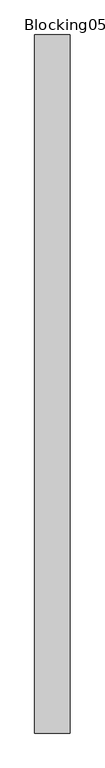
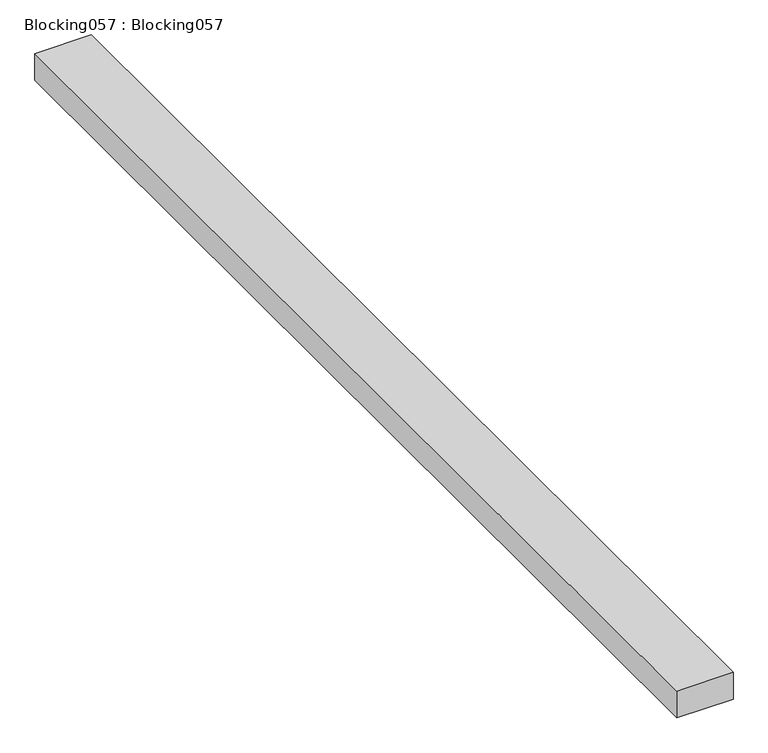
"""IFC4 building model written with IfcOpenShell, lengths in millimetres: proxy geometry, Blocking057 : Blocking057."""

from ifc_helpers import new_model, si_unit, frame, origin, place, context, project, spatial, polyline, outline, extrude, source, transform, mapped, element, save


def blocking057_blocking057_3770e6a9(model_context):
    return source(origin(), model_context, "Body", "SweptSolid", [
        extrude(outline(polyline([(-9298.3737014, 7982.1531721), (-9399.9737014, 7982.1531721), (-9399.9737014, 9982.1531721), (-9298.3737014, 9982.1531721), (-9298.3737014, 7982.1531721)])), frame((0.0, 0.0, 40004.7460083), z_axis=(0.0, 0.0, 1.0), x_axis=(1.0, 0.0, 0.0)), (0.0, 0.0, 1.0), 50.8),
    ])


if __name__ == "__main__":
    model = new_model("IFC4")
    model_context = context("Model", 3, world=origin())
    ifc_project = project(units=[si_unit("LENGTHUNIT", "METRE", prefix="MILLI")], contexts=[model_context])
    site = spatial("IfcSite", under=ifc_project)
    building = spatial("IfcBuilding", under=site)
    placement = place(None, origin())
    blocking057_blocking057_shape = blocking057_blocking057_3770e6a9(model_context)
    element("IfcBuildingElementProxy", 1, Name="Blocking057 : Blocking057", ObjectType="Blocking057 : Blocking057", at=placement, inside=building, context=model_context, shape_type="MappedRepresentation", body=[
        mapped(blocking057_blocking057_shape, transform((0.0, 0.0, 0.0), x_axis=(1.0, 0.0, 0.0), y_axis=(0.0, 1.0, 0.0), z_axis=(0.0, 0.0, 1.0))),
    ])
    save(model, "model.ifc")

# Revit data of these elements
# Type "Blocking057 : Blocking057"
#   NameOverride = "Blocking057"
# Element 1 (IfcBuildingElementProxy, "Blocking057 : Blocking057")
#   Materials on its faces: "WOOD BLOCKING AS REQUIRED"
# Materials
#   "WOOD BLOCKING AS REQUIRED": class "Unassigned", colour RGB 166 124 85, transparency 0, Cost = 0
